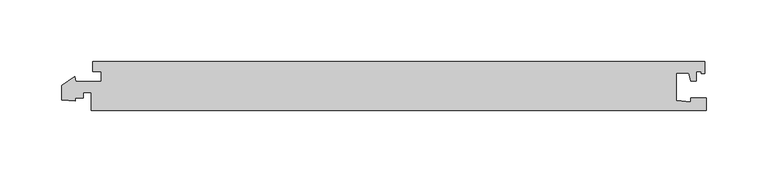
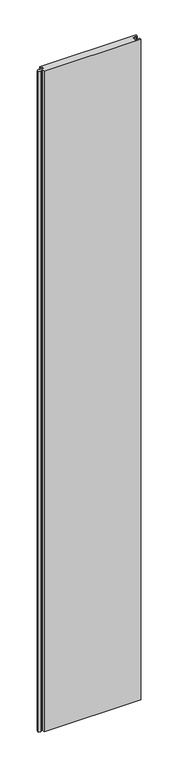
"""IFC4 building model written with IfcOpenShell, lengths in millimetres: proxy geometry, Generic Models 5:Generic Models 5:321804:Generic Models 5:321804 : Generic Models 5:Generic Models 5:321804:7 : Generic Models 5:Generic Models 5:321804:Generic Models 5:321804 : Generic Models 5:Generic Models 5:321804:300761."""

from ifc_helpers import new_model, si_unit, frame, origin, place, context, project, spatial, polyline, outline, extrude, source, transform, mapped, element, save


def generic_models_1586af21(model_context):
    return source(origin(), model_context, "Body", "SweptSolid", [
        extrude(outline(polyline([(592720.2261126, -579052.1037319), (592709.8677824, -579052.1037319), (592709.8677824, -579074.5995222), (592721.8677824, -579075.6493861), (592721.8677824, -579072.4037319), (592734.6177824, -579072.4037319), (592734.6177824, -579082.6037319), (592234.6177824, -579082.6037319), (592234.6177824, -579068.1037319), (592227.9927824, -579068.1037319), (592227.9927824, -579072.4037319), (592221.3677824, -579072.4037319), (592221.3677824, -579075.1037319), (592210.3677824, -579074.1413566), (592210.3677824, -579062.2832156), (592221.0492843, -579055.1758504), (592222.101757, -579059.1037319), (592242.8177824, -579059.1037319), (592242.8177824, -579051.1037319), (592235.8677824, -579051.1037319), (592235.8677824, -579042.6037319), (592733.3677824, -579042.6037319), (592733.3677824, -579052.6037319), (592730.3677824, -579052.6037319), (592730.3677824, -579051.1037319), (592726.4177824, -579051.1037319), (592726.4177824, -579058.6037319), (592721.9677824, -579058.6037319), (592720.2261126, -579052.1037319)])), frame((0.0, 0.0, 42.1702614), z_axis=(0.0, 0.0, 1.0), x_axis=(1.0, 0.0, 0.0)), (0.0, 0.0, 1.0), 3608.6890331),
    ])


if __name__ == "__main__":
    model = new_model("IFC4")
    model_context = context("Model", 3, world=origin())
    ifc_project = project(units=[si_unit("LENGTHUNIT", "METRE", prefix="MILLI")], contexts=[model_context])
    site = spatial("IfcSite", under=ifc_project)
    building = spatial("IfcBuilding", under=site)
    placement = place(None, origin())
    generic_models_shape = generic_models_1586af21(model_context)
    element("IfcBuildingElementProxy", 1, Name="Generic Models 5:Generic Models 5:321804:Generic Models 5:321804 : Generic Models 5:Generic Models 5:321804:7 : Generic Models 5:Generic Models 5:321804:Generic Models 5:321804 : Generic Models 5:Generic Models 5:321804:300761", ObjectType="Generic Models 5:Generic Models 5:321804:Generic Models 5:321804 : Generic Models 5:Generic Models 5:321804:7 : Generic Models 5:Generic Models 5:321804:Generic Models 5:321804 : Generic Models 5:Generic Models 5:321804:300761", at=placement, inside=building, context=model_context, shape_type="MappedRepresentation", body=[
        mapped(generic_models_shape, transform((0.0, 0.0, 0.0), x_axis=(1.0, 0.0, 0.0), y_axis=(0.0, 1.0, 0.0), z_axis=(0.0, 0.0, 1.0))),
    ])
    save(model, "model.ifc")

# Revit data of these elements
# Type "Generic Models 5:Generic Models 5:321804:Generic Models 5:321804 : Generic Models 5:Generic Models 5:321804:7 : Generic Models 5:Generic Models 5:321804:Generic Models 5:321804 : Generic Models 5:Generic Models 5:321804:300761"
#   NameOverride = "Generic Models 5:Generic Models 5:321804:Generic Models 5:321804 : Generic Models 5:Generic Models 5:321804:300761"
#   ObjectTypeOverride = "Generic Models 5:321804 : Generic Models 5:Generic Models 5:321804"
#   Reference = "Generic Models 5"
#   Tag = "300761"
# Element 1 (IfcBuildingElementProxy, "Generic Models 5:Generic Models 5:321804:Generic Models 5:321804 : Generic Models 5:Generic Models 5:321804:7 : Generic Models 5:Generic Models 5:321804:Generic Models 5:321804 : Generic Models 5:Generic Models 5:321804:300761")
#   Materials on its faces: "POLYCARBONATE PANEL - ARCOPLUS 547"
# Materials
#   "POLYCARBONATE PANEL - ARCOPLUS 547": class "Unassigned", colour RGB 202 225 249, transparency 0.45, Cost = 0
